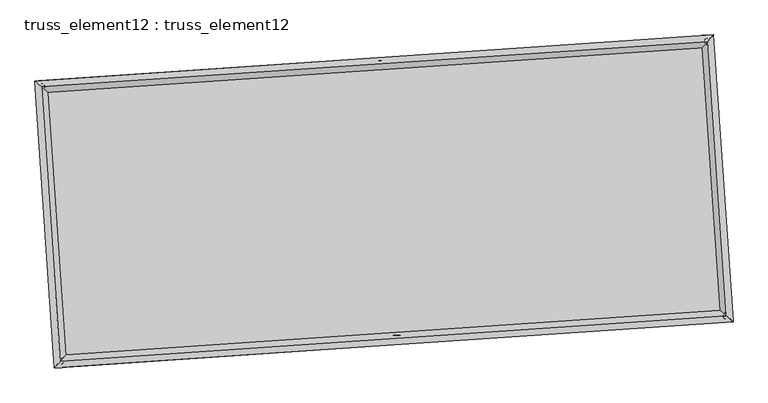
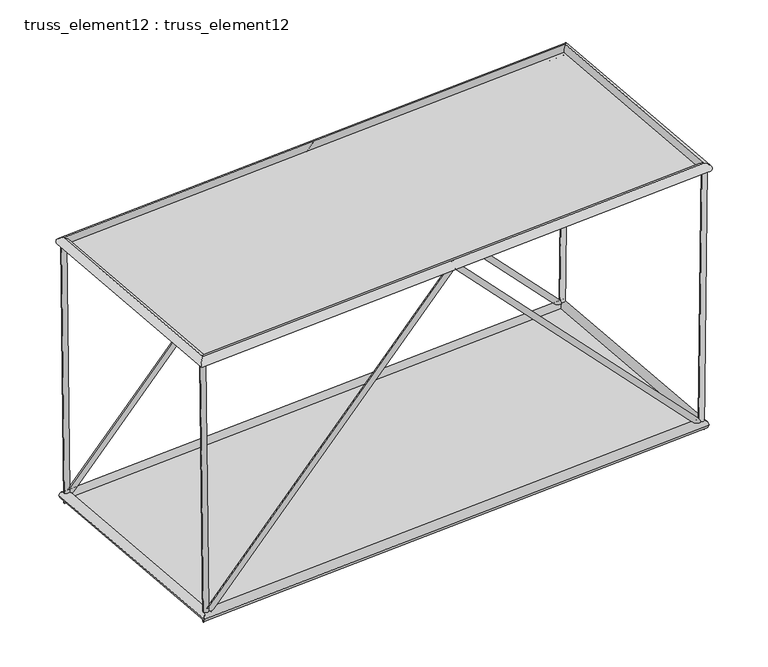
"""IFC4 building model written with IfcOpenShell, lengths in millimetres: plate geometry, truss_element12 : truss_element12."""

from ifc_helpers import new_model, si_unit, frame, origin, origin_with_axes, place, context, project, spatial, polyline, circle_curve, ellipse_curve, outline, extrude, source, transform, mapped, element, save
from ifc_brep_helpers import plane_surface, cylinder_surface, advanced_brep


def truss_element12_truss_element12_f74dbc9f(model_context):
    return source(origin(), model_context, "Body", "SolidModel", [
        advanced_brep(
        [(-3723.9375592, 2272.2012616, 5000.2403686), (-3823.0339641, 2258.8404944, 4999.0603521), (-3666.3858201, 2276.1254959, 122.6805118), (-3762.6010627, 2262.9611842, -122.6805118), (1064.2598437, 2598.6902408, 5071.7652226), (1064.6999756, 2592.1164917, 4927.5226657), (5793.8507749, 2921.1830676, 122.672987), (5890.9102021, 2921.1974209, -122.672987), (5852.4493048, 2925.1786786, 5000.2382655), (5952.4418571, 2925.3930306, 4999.0367904)],
        [
            (0, 1, circle_curve(frame((-3773.4857617, 2265.520878, 4999.6503604), z_axis=(-0.011798464054871819, -0.0008044924137411783, 0.9999300720739938), x_axis=(-0.13360782212564323, 0.9910339766144194, -0.0007791422546549884)), 50.0)),
            (1, 0, circle_curve(frame((-3773.4857617, 2265.520878, 4999.6503604), z_axis=(-0.011798464054871819, -0.0008044924137411783, 0.9999300720739938), x_axis=(-0.13360782212564323, 0.9910339766144194, -0.0007791422546549884)), 50.0)),
            (0, 2),
            (2, 3, ellipse_curve(frame((-3714.4934414, 2269.54334, 0.0), z_axis=(-0.9279553876166271, -0.06327375039291133, 0.36728086133705756), x_axis=(0.3664300170520614, 0.02498546993188102, 0.9301100842886874)), 132.1861236, 50.0)),
            (3, 1),
            (3, 2, ellipse_curve(frame((-3714.4934414, 2269.54334, 0.0), z_axis=(-0.9279553876166271, -0.06327375039291133, 0.36728086133705756), x_axis=(0.3664300170520614, 0.02498546993188102, 0.9301100842886874)), 132.1861236, 50.0)),
            (2, 4),
            (4, 5, ellipse_curve(frame((1064.4799096, 2595.4033663, 4999.6439441), z_axis=(-0.997683394506372, -0.06802823812175422, 5.607399430256163e-05), x_axis=(-5.5944093067282144e-05, -3.814615042673666e-06, -0.9999999984278535)), 72.2783214, 50.0)),
            (5, 3),
            (5, 4, ellipse_curve(frame((1064.4799096, 2595.4033663, 4999.6439441), z_axis=(-0.997683394506372, -0.06802823812175422, 5.607399430256163e-05), x_axis=(-5.5944093067282144e-05, -3.814615042673666e-06, -0.9999999984278535)), 72.2783214, 50.0)),
            (4, 6),
            (6, 7, ellipse_curve(frame((5842.3804885, 2921.1902443, 0.0), z_axis=(-0.9280153260656241, -0.06327783736790117, -0.36712868300550267), x_axis=(-0.36627819125742656, -0.024975117508088982, 0.9301701619137465)), 132.1694786, 50.0)),
            (7, 5),
            (7, 6, ellipse_curve(frame((5842.3804885, 2921.1902443, 0.0), z_axis=(-0.9280153260656241, -0.06327783736790117, -0.36712868300550267), x_axis=(-0.36627819125742656, -0.024975117508088982, 0.9301701619137465)), 132.1694786, 50.0)),
            (8, 9, circle_curve(frame((5902.4455809, 2925.2858546, 4999.6375279), z_axis=(0.012013018486840912, 0.0008191220648592267, 0.9999275055852187), x_axis=(-0.0021532060735693225, 0.999997367177233, -0.0007933109144987253)), 50.0)),
            (9, 8, circle_curve(frame((5902.4455809, 2925.2858546, 4999.6375279), z_axis=(0.012013018486840912, 0.0008191220648592267, 0.9999275055852187), x_axis=(-0.0021532060735693225, 0.999997367177233, -0.0007933109144987253)), 50.0)),
            (6, 8),
            (9, 7),
        ],
        [
            plane_surface(frame((-3773.4857617, 2315.5208618, 4999.6905878), z_axis=(-0.011798464054872752, -0.0008044924137361026, 0.9999300720739939), x_axis=(0.9999303957005937, -9.492435539826266e-06, 0.011798460236310156))),
            cylinder_surface(frame((-3773.4857617, 2265.520878, 4999.6503604), z_axis=(-0.011798464054871819, -0.0008044924137411783, 0.9999300720739938), x_axis=(-0.13360782212564323, 0.9910339766144194, -0.0007791422546549884)), 50.0),
            cylinder_surface(frame((-3714.4934414, 2269.54334, 0.0), z_axis=(-0.6902081933695349, -0.0470626729788961, -0.7220787731388068), x_axis=(-0.020416755864474615, 0.9987520451432434, -0.04557969287038922)), 50.0),
            cylinder_surface(frame((1064.4799096, 2595.4033663, 4999.6439441), z_axis=(-0.6901273969450558, -0.04705716377784709, 0.7221563537926025), x_axis=(-0.11534920316499872, 0.9922789624338372, -0.045574357268395246)), 50.0),
            plane_surface(frame((5902.4455809, 2875.2858714, 4999.678487), z_axis=(0.012013018486842117, 0.0008191220648596662, 0.9999275055852188), x_axis=(0.9999278410899632, -9.84083861155227e-06, -0.012013014456126566))),
            cylinder_surface(frame((5842.3804885, 2921.1902443, 0.0), z_axis=(-0.012013018486840915, -0.000819122064859227, -0.9999275055852189), x_axis=(-0.0021532060735693225, 0.999997367177233, -0.0007933109144987253)), 50.0),
        ],
        [
            (0, [[1, 2]]),
            (1, [[-1, 3, 4, 5]]),
            (1, [[-2, -5, 6, -3]]),
            (2, [[-4, 7, 8, 9]]),
            (2, [[-6, -9, 10, -7]]),
            (3, [[-8, 11, 12, 13]]),
            (3, [[-10, -13, 14, -11]]),
            (4, [[15, 16]]),
            (5, [[-12, 17, -16, 18]]),
            (5, [[-14, -18, -15, -17]]),
        ],
    ),
        advanced_brep(
        [(-3451.8246063, -1718.5323227, 5000.2403686), (-3550.9210112, -1731.8930899, 4999.0603521), (-3394.2728672, -1714.6080884, 122.6805118), (-3490.4881098, -1727.7724001, -122.6805118), (1336.3727966, -1392.0433435, 5071.7652226), (1336.8129285, -1398.6170926, 4927.5226657), (6065.9637278, -1069.5505167, 122.672987), (6163.023155, -1069.5361634, -122.672987), (6124.5622577, -1065.5549057, 5000.2382655), (6224.55481, -1065.3405537, 4999.0367904)],
        [
            (0, 1, circle_curve(frame((-3501.3728088, -1725.2127063, 4999.6503604), z_axis=(-0.01179846405487153, -0.0008044924137411652, 0.9999300720739936), x_axis=(-0.133607822125643, 0.9910339766144194, -0.0007791422546549605)), 50.0)),
            (1, 0, circle_curve(frame((-3501.3728088, -1725.2127063, 4999.6503604), z_axis=(-0.01179846405487153, -0.0008044924137411652, 0.9999300720739936), x_axis=(-0.133607822125643, 0.9910339766144194, -0.0007791422546549605)), 50.0)),
            (0, 2),
            (2, 3, ellipse_curve(frame((-3442.3804885, -1721.1902443, 0.0), z_axis=(-0.927955387616627, -0.06327375039291126, 0.3672808613370578), x_axis=(0.3664300170520616, 0.024985469931880992, 0.9301100842886872)), 132.1861236, 50.0)),
            (3, 1),
            (3, 2, ellipse_curve(frame((-3442.3804885, -1721.1902443, 0.0), z_axis=(-0.927955387616627, -0.06327375039291126, 0.3672808613370578), x_axis=(0.3664300170520616, 0.024985469931880992, 0.9301100842886872)), 132.1861236, 50.0)),
            (2, 4),
            (4, 5, ellipse_curve(frame((1336.5928625, -1395.330218, 4999.6439441), z_axis=(-0.997683394506372, -0.06802823812175413, 5.6073994302962844e-05), x_axis=(-5.5944093067589644e-05, -3.8146150427121027e-06, -0.9999999984278536)), 72.2783214, 50.0)),
            (5, 3),
            (5, 4, ellipse_curve(frame((1336.5928625, -1395.330218, 4999.6439441), z_axis=(-0.997683394506372, -0.06802823812175413, 5.6073994302962844e-05), x_axis=(-5.5944093067589644e-05, -3.8146150427121027e-06, -0.9999999984278536)), 72.2783214, 50.0)),
            (4, 6),
            (6, 7, ellipse_curve(frame((6114.4934414, -1069.54334, 0.0), z_axis=(-0.9280153260656242, -0.063277837367901, -0.3671286830055023), x_axis=(-0.3662781912574264, -0.024975117508088944, 0.9301701619137466)), 132.1694786, 50.0)),
            (7, 5),
            (7, 6, ellipse_curve(frame((6114.4934414, -1069.54334, 0.0), z_axis=(-0.9280153260656242, -0.063277837367901, -0.3671286830055023), x_axis=(-0.3662781912574264, -0.024975117508088944, 0.9301701619137466)), 132.1694786, 50.0)),
            (8, 9, circle_curve(frame((6174.5585339, -1065.4477297, 4999.6375279), z_axis=(0.01201301848684124, 0.0008191220648592048, 0.9999275055852187), x_axis=(-0.00215320607356917, 0.999997367177233, -0.0007933109144987045)), 50.0)),
            (9, 8, circle_curve(frame((6174.5585339, -1065.4477297, 4999.6375279), z_axis=(0.01201301848684124, 0.0008191220648592048, 0.9999275055852187), x_axis=(-0.00215320607356917, 0.999997367177233, -0.0007933109144987045)), 50.0)),
            (6, 8),
            (9, 7),
        ],
        [
            plane_surface(frame((-3501.3728088, -1675.2127225, 4999.6905878), z_axis=(-0.011798464054872752, -0.000804492413736107, 0.9999300720739939), x_axis=(0.9999303957005937, -9.492435539826266e-06, 0.011798460236310156))),
            cylinder_surface(frame((-3501.3728088, -1725.2127063, 4999.6503604), z_axis=(-0.01179846405487153, -0.0008044924137411652, 0.9999300720739936), x_axis=(-0.133607822125643, 0.9910339766144194, -0.0007791422546549605)), 50.0),
            cylinder_surface(frame((-3442.3804885, -1721.1902443, 0.0), z_axis=(-0.6902081933695352, -0.04706267297889607, -0.7220787731388064), x_axis=(-0.020416755864474608, 0.9987520451432436, -0.045579692870389196)), 50.0),
            cylinder_surface(frame((1336.5928625, -1395.330218, 4999.6439441), z_axis=(-0.6901273969450555, -0.04705716377784698, 0.7221563537926026), x_axis=(-0.11534920316499851, 0.9922789624338372, -0.045574357268395156)), 50.0),
            plane_surface(frame((6174.5585339, -1115.4477129, 4999.678487), z_axis=(0.012013018486842117, 0.0008191220648596683, 0.9999275055852188), x_axis=(0.9999278410899632, -9.840838612440448e-06, -0.012013014456126566))),
            cylinder_surface(frame((6114.4934414, -1069.54334, 0.0), z_axis=(-0.012013018486841243, -0.0008191220648592051, -0.9999275055852189), x_axis=(-0.00215320607356917, 0.999997367177233, -0.0007933109144987045)), 50.0),
        ],
        [
            (0, [[1, 2]]),
            (1, [[-1, 3, 4, 5]]),
            (1, [[-2, -5, 6, -3]]),
            (2, [[-4, 7, 8, 9]]),
            (2, [[-6, -9, 10, -7]]),
            (3, [[-8, 11, 12, 13]]),
            (3, [[-10, -13, 14, -11]]),
            (4, [[15, 16]]),
            (5, [[-12, 17, -16, 18]]),
            (5, [[-14, -18, -15, -17]]),
        ],
    ),
        advanced_brep(
        [(-3501.3761785, -1725.2164412, 4909.6503604), (-3501.369439, -1725.2089715, 5089.6503603), (-3773.4819161, 2265.5176351, 5089.6503603), (-3773.4896072, 2265.5241208, 4909.6503604), (5902.4424488, 2925.2821359, 5089.6375279), (5902.4487131, 2925.2895732, 4909.637528), (6174.5549259, -1065.4444707, 5089.6375279), (6174.5621418, -1065.4509888, 4909.637528)],
        [
            (0, 1, ellipse_curve(frame((-3501.3728088, -1725.2127063, 4999.6503604), z_axis=(-0.7535719234048426, 0.6573654662781203, 9.356088950770169e-07), x_axis=(-0.6573654662774605, -0.7535719234054181, 9.356088950769949e-07)), 127.2792206, 90.0)),
            (1, 2),
            (2, 3, ellipse_curve(frame((-3773.4857617, 2265.520878, 4999.6503604), z_axis=(-0.6573654662774606, -0.7535719234054181, 9.356088950769758e-07), x_axis=(0.7535719234048427, -0.6573654662781201, -9.356088950769975e-07)), 127.2792206, 90.0)),
            (3, 0),
            (1, 0, ellipse_curve(frame((-3501.3728088, -1725.2127063, 4999.6503604), z_axis=(-0.7535719234048426, 0.6573654662781203, 9.356088950770169e-07), x_axis=(-0.6573654662774605, -0.7535719234054181, 9.356088950769949e-07)), 127.2792206, 90.0)),
            (3, 2, ellipse_curve(frame((-3773.4857617, 2265.520878, 4999.6503604), z_axis=(-0.6573654662774606, -0.7535719234054181, 9.356088950769758e-07), x_axis=(0.7535719234048427, -0.6573654662781201, -9.356088950769975e-07)), 127.2792206, 90.0)),
            (2, 4),
            (4, 5, ellipse_curve(frame((5902.4455809, 2925.2858546, 4999.6375279), z_axis=(-0.7535719234048426, 0.6573654662781203, 9.356088950769785e-07), x_axis=(-0.657365466277461, -0.7535719234054179, 9.356088950769951e-07)), 127.2792206, 90.0)),
            (5, 3),
            (5, 4, ellipse_curve(frame((5902.4455809, 2925.2858546, 4999.6375279), z_axis=(-0.7535719234048426, 0.6573654662781203, 9.356088950769785e-07), x_axis=(-0.657365466277461, -0.7535719234054179, 9.356088950769951e-07)), 127.2792206, 90.0)),
            (4, 6),
            (6, 7, ellipse_curve(frame((6174.5585339, -1065.4477297, 4999.6375279), z_axis=(0.6573654662774608, 0.7535719234054181, -9.356088950770147e-07), x_axis=(-0.7535719234048427, 0.6573654662781202, 9.356088950769979e-07)), 127.2792206, 90.0)),
            (7, 5),
            (7, 6, ellipse_curve(frame((6174.5585339, -1065.4477297, 4999.6375279), z_axis=(0.6573654662774608, 0.7535719234054181, -9.356088950770147e-07), x_axis=(-0.7535719234048427, 0.6573654662781202, 9.356088950769979e-07)), 127.2792206, 90.0)),
            (6, 1),
            (0, 7),
        ],
        [
            cylinder_surface(frame((-3501.3728088, -1725.2127063, 4999.6503604), z_axis=(0.06802823822870396, -0.9976833960748764, 0.0), x_axis=(-0.9976833952696048, -0.06802823817379555, 4.017813848825568e-05)), 90.0),
            cylinder_surface(frame((-3773.4857617, 2265.520878, 4999.6503604), z_axis=(-0.997683396074003, -0.06802823822864602, 1.3231507884947808e-06), x_axis=(-0.0680282381260622, 0.9976833953252674, 3.8854987700759686e-05)), 90.0),
            cylinder_surface(frame((5902.4455809, 2925.2858546, 4999.6375279), z_axis=(-0.06802823822870392, 0.9976833960748763, 0.0), x_axis=(0.9976833953721886, 0.0680282381807903, 3.753183691326367e-05)), 90.0),
            cylinder_surface(frame((6174.5585339, -1065.4477297, 4999.6375279), z_axis=(0.997683396074003, 0.06802823822864555, -1.3231507884948084e-06), x_axis=(0.06802823822864554, -0.9976833953182727, 3.8854987700759665e-05)), 90.0),
        ],
        [
            (0, [[1, 2, 3, 4]]),
            (0, [[5, -4, 6, -2]]),
            (1, [[-3, 7, 8, 9]]),
            (1, [[-6, -9, 10, -7]]),
            (2, [[-8, 11, 12, 13]]),
            (2, [[-10, -13, 14, -11]]),
            (3, [[-12, 15, -1, 16]]),
            (3, [[-14, -16, -5, -15]]),
        ],
    ),
        advanced_brep(
        [(-3358.7115243, -1625.2761972, 0.0), (-3526.0494527, -1817.1042913, 0.0), (-3810.4074885, 2353.2123043, 0.0), (-3618.5793943, 2185.8743758, 0.0), (5926.0494527, 3017.1042913, 0.0), (5758.7115243, 2825.2761972, 0.0), (6210.4074885, -1153.2123043, 0.0), (6018.5793943, -985.8743758, 0.0)],
        [
            (0, 1, ellipse_curve(frame((-3442.3804885, -1721.1902443, 0.0), z_axis=(-0.7535719234054595, 0.6573654662780791, 0.0), x_axis=(-0.6573654662780791, -0.7535719234054593, 0.0)), 127.2792206, 90.0)),
            (1, 2),
            (2, 3, ellipse_curve(frame((-3714.4934414, 2269.54334, 0.0), z_axis=(-0.6573654662780787, -0.7535719234054598, 0.0), x_axis=(0.7535719234054598, -0.6573654662780787, 0.0)), 127.2792206, 90.0)),
            (3, 0),
            (1, 0, ellipse_curve(frame((-3442.3804885, -1721.1902443, 0.0), z_axis=(-0.7535719234054595, 0.6573654662780791, 0.0), x_axis=(-0.6573654662780791, -0.7535719234054593, 0.0)), 127.2792206, 90.0)),
            (3, 2, ellipse_curve(frame((-3714.4934414, 2269.54334, 0.0), z_axis=(-0.6573654662780787, -0.7535719234054598, 0.0), x_axis=(0.7535719234054598, -0.6573654662780787, 0.0)), 127.2792206, 90.0)),
            (2, 4),
            (4, 5, ellipse_curve(frame((5842.3804885, 2921.1902443, 0.0), z_axis=(-0.7535719234054595, 0.6573654662780789, 0.0), x_axis=(-0.657365466278079, -0.7535719234054594, 0.0)), 127.2792206, 90.0)),
            (5, 3),
            (5, 4, ellipse_curve(frame((5842.3804885, 2921.1902443, 0.0), z_axis=(-0.7535719234054595, 0.6573654662780789, 0.0), x_axis=(-0.657365466278079, -0.7535719234054594, 0.0)), 127.2792206, 90.0)),
            (4, 6),
            (6, 7, ellipse_curve(frame((6114.4934414, -1069.54334, 0.0), z_axis=(0.6573654662780792, 0.7535719234054592, 0.0), x_axis=(-0.7535719234054591, 0.6573654662780795, 0.0)), 127.2792206, 90.0)),
            (7, 5),
            (7, 6, ellipse_curve(frame((6114.4934414, -1069.54334, 0.0), z_axis=(0.6573654662780792, 0.7535719234054592, 0.0), x_axis=(-0.7535719234054591, 0.6573654662780795, 0.0)), 127.2792206, 90.0)),
            (6, 1),
            (0, 7),
        ],
        [
            cylinder_surface(frame((-3442.3804885, -1721.1902443, 0.0), z_axis=(0.06802823822870316, -0.9976833960748764, 0.0), x_axis=(-0.9976833960748764, -0.06802823822870316, 0.0)), 90.0),
            cylinder_surface(frame((-3714.4934414, 2269.54334, 0.0), z_axis=(-0.9976833960748763, -0.06802823822870475, 0.0), x_axis=(-0.06802823822870475, 0.9976833960748763, 0.0)), 90.0),
            cylinder_surface(frame((5842.3804885, 2921.1902443, 0.0), z_axis=(-0.06802823822870278, 0.9976833960748767, 0.0), x_axis=(0.9976833960748767, 0.06802823822870278, 0.0)), 90.0),
            cylinder_surface(frame((6114.4934414, -1069.54334, 0.0), z_axis=(0.9976833960748765, 0.0680282382287038, 0.0), x_axis=(0.0680282382287038, -0.9976833960748765, 0.0)), 90.0),
        ],
        [
            (0, [[1, 2, 3, 4]]),
            (0, [[5, -4, 6, -2]]),
            (1, [[-3, 7, 8, 9]]),
            (1, [[-6, -9, 10, -7]]),
            (2, [[-8, 11, 12, 13]]),
            (2, [[-10, -13, 14, -11]]),
            (3, [[-12, 15, -1, 16]]),
            (3, [[-14, -16, -5, -15]]),
        ],
    ),
        extrude(outline(polyline([(-3442.3804885, -1721.1902443), (-3714.4934414, 2269.54334), (5842.3804885, 2921.1902443), (6114.4934414, -1069.54334), (-3442.3804885, -1721.1902443)])), origin_with_axes(), (0.0, 0.0, 1.0), 20.0),
        extrude(outline(polyline([(-1999.9999999, 4849.1993456), (2000.0, 4849.1993456), (2000.0000001, -4849.1993455), (-1999.9999999, -4849.1993456), (-1999.9999999, 4849.1993456)])), frame((1200.5363861, 600.0365741, 4999.6439441), z_axis=(1.3200855721846371e-06, 9.001161705222004e-08, 0.9999999999991248), x_axis=(-0.06802823822870295, 0.9976833960748764, 0.0)), (0.0, 0.0, 1.0), 20.0),
    ])


if __name__ == "__main__":
    model = new_model("IFC4")
    model_context = context("Model", 3, world=origin())
    ifc_project = project(units=[si_unit("LENGTHUNIT", "METRE", prefix="MILLI")], contexts=[model_context])
    site = spatial("IfcSite", under=ifc_project)
    building = spatial("IfcBuilding", under=site)
    placement = place(None, origin())
    truss_element12_truss_element12_shape = truss_element12_truss_element12_f74dbc9f(model_context)
    element("IfcPlate", 1, ObjectType="truss_element12 : truss_element12", at=placement, inside=building, context=model_context, shape_type="MappedRepresentation", body=[
        mapped(truss_element12_truss_element12_shape, transform((0.0, 0.0, 0.0), x_axis=(1.0, 0.0, 0.0), y_axis=(0.0, 1.0, 0.0), z_axis=(0.0, 0.0, 1.0))),
    ])
    save(model, "model.ifc")

# Revit data of these elements
# Type "truss_element12 : truss_element12"
#   steellbar1 = 90 mm
#   steelbar2 = 50 mm
#   offset1 = 5000 mm
#   M = Default Roof
# Element 1 (IfcPlate, "truss_element12 : truss_element12")
#   Materials on its faces: "Default Roof"
# Materials
#   "Default Roof": class "Miscellaneous", colour RGB 0 127 0, transparency 0, Comments = "Rendering appearance not upgraded Rendering appearance not upgraded ", Cost = 0
